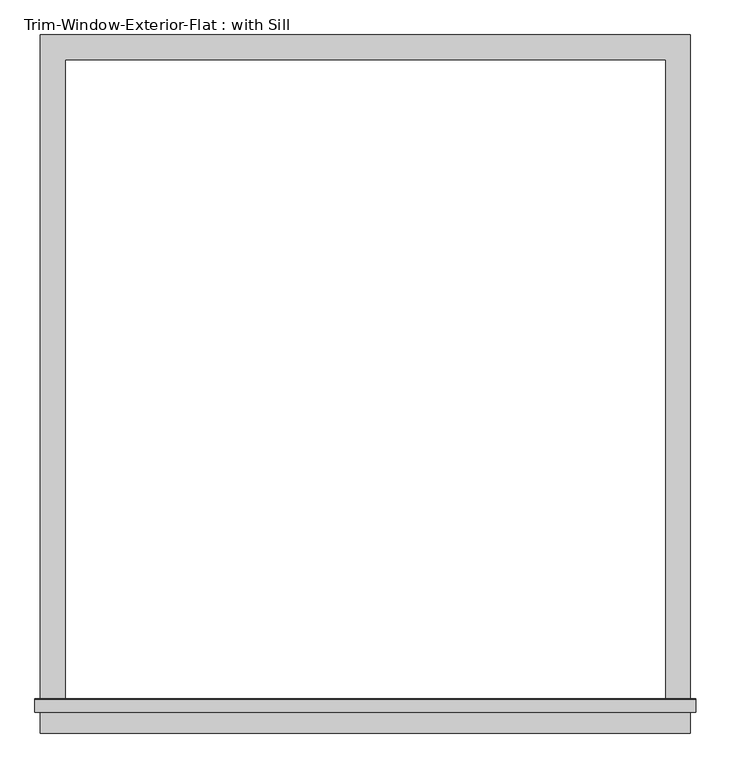
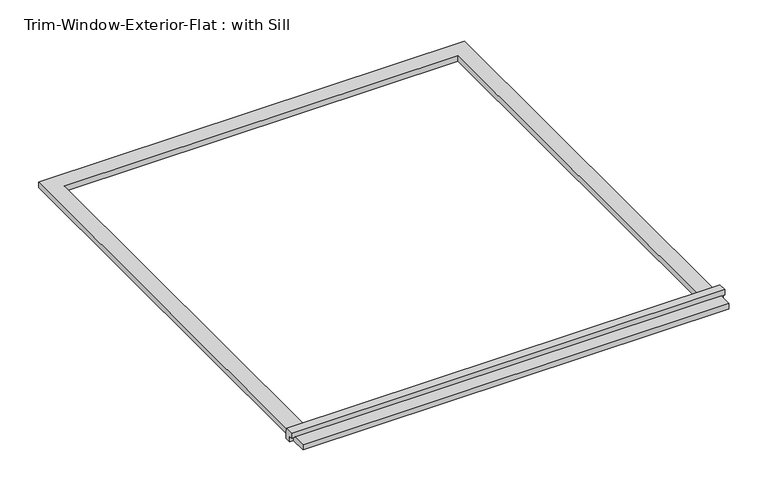
"""IFC4 building model written with IfcOpenShell, lengths in millimetres: proxy geometry, Trim-Window-Exterior-Flat : with Sill."""

from ifc_helpers import new_model, si_unit, frame, origin, origin_with_axes, place, context, project, spatial, polyline, outline, extrude, source, transform, mapped, element, save


def trim_window_exterior_flat_with_sill_8d50fb7e(model_context):
    return source(origin(), model_context, "Body", "SweptSolid", [
        extrude(outline(polyline([(749.3, -1495.3823709), (749.3, -1552.5323709), (-749.3, -1552.5323709), (-749.3, -1495.3823709), (749.3, -1495.3823709)])), origin_with_axes(), (0.0, 0.0, 1.0), 19.05),
        extrude(outline(polyline([(-1504.95, 38.1), (-1475.6580645, 38.1), (-1473.2, 19.05), (-1473.2, 0.0), (-1495.3823709, 0.0), (-1495.3823709, 19.05), (-1504.95, 19.05), (-1504.95, 38.1)])), frame((-762.0, 0.0, 0.0), z_axis=(1.0, 0.0, 0.0), x_axis=(0.0, 1.0, 0.0)), (0.0, 0.0, 1.0), 1524.0),
        extrude(outline(polyline([(-749.3, 57.15), (749.3, 57.15), (749.3, -1473.2), (692.15, -1473.2), (692.15, 0.0), (-692.15, 0.0), (-692.15, -1473.2), (-749.3, -1473.2), (-749.3, 57.15)])), origin_with_axes(), (0.0, 0.0, 1.0), 19.05),
    ])


if __name__ == "__main__":
    model = new_model("IFC4")
    model_context = context("Model", 3, world=origin())
    ifc_project = project(units=[si_unit("LENGTHUNIT", "METRE", prefix="MILLI")], contexts=[model_context])
    site = spatial("IfcSite", under=ifc_project)
    building = spatial("IfcBuilding", under=site)
    placement = place(None, origin())
    trim_window_exterior_flat_with_sill_shape = trim_window_exterior_flat_with_sill_8d50fb7e(model_context)
    element("IfcBuildingElementProxy", 1, Name="Trim-Window-Exterior-Flat : with Sill", ObjectType="Trim-Window-Exterior-Flat : with Sill", at=placement, inside=building, context=model_context, shape_type="MappedRepresentation", body=[
        mapped(trim_window_exterior_flat_with_sill_shape, transform((0.0, 0.0, 0.0), x_axis=(1.0, 0.0, 0.0), y_axis=(0.0, 1.0, 0.0), z_axis=(0.0, 0.0, 1.0))),
    ])
    save(model, "model.ifc")

# Revit data of these elements
# Type "Trim-Window-Exterior-Flat : with Sill"
#   Trim Width = 0' - 2 1/4"
#   Trim Thickness_Picture Frame = 0' - 1 1/4"
#   Trim Thickness_with Sill = 0' - 0 3/4"
#   Sill Thickness = 0' - 1 1/4"
#   Opening Width [instance default] = 2' - 0"
#   Opening Height [instance default] = 3' - 0"
#   Default Elevation = 4' - 0"
#   Sill = yes
#   Picture Frame = no
#   Trim Material [instance default] = none
# Element 1 (IfcBuildingElementProxy, "Trim-Window-Exterior-Flat : with Sill")
#   Opening Width = 4' - 6 1/2"
#   Opening Height = 4' - 10"
#   Trim Material = 1X WOOD COMPOSITE TRIM
#   Materials on its faces: "1X WOOD COMPOSITE TRIM"
# Materials
#   "1X WOOD COMPOSITE TRIM": class "Generic", colour RGB 88 61 61, transparency 0, Cost = 0
